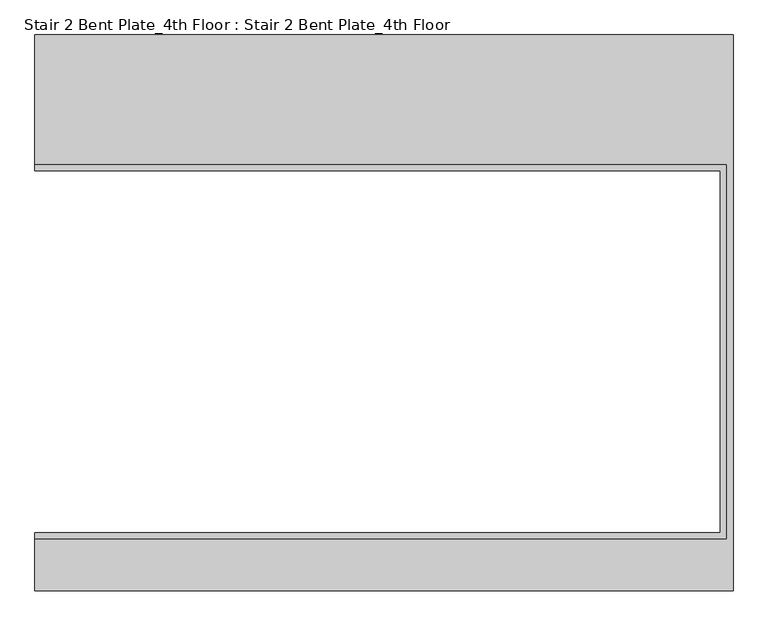
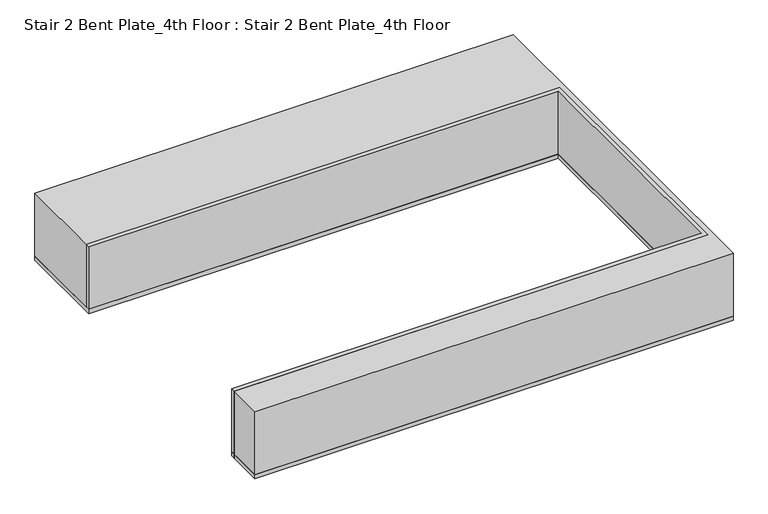
"""IFC4 building model written with IfcOpenShell, lengths in millimetres: proxy geometry, Stair 2 Bent Plate_4th Floor : Stair 2 Bent Plate_4th Floor."""

import ifcopenshell
import ifcopenshell.guid

model = None  # the IFC model being written
_history = None  # IfcOwnerHistory: only IFC2X3 demands one
_inside = {}  # id of a spatial element -> (the spatial element, [elements in it])
_under = {}  # id of a project, library or spatial element -> (it, [spatial elements below it])
_declared = {}  # id of a project -> (the project, [libraries it declares])
_typed = {}  # id of a type object -> (the type object, [elements of that type])
_made_of = {}  # id of a material, layer set ... -> (it, [elements and type objects made of it])


def new_model(schema):
    """Start an empty IFC model of exactly this schema.

    Asked for "IFC4X3", IfcOpenShell would pick the latest addendum, in which some entities
    have other attributes; the version numbers below select the first issue.
    IFC2X3 requires an IfcOwnerHistory on every rooted entity: one is made here for all.
    """
    global model, _history
    if schema == "IFC4X3":
        model = ifcopenshell.file(schema_version=(4, 3, 0, 0))
    else:
        model = ifcopenshell.file(schema=schema)
    _inside.clear()
    _under.clear()
    _declared.clear()
    _typed.clear()
    _made_of.clear()
    _history = None
    if model.schema == "IFC2X3":
        org = make("IfcOrganization", Name="unknown")
        user = make(
            "IfcPersonAndOrganization",
            ThePerson=make("IfcPerson", FamilyName="unknown"),
            TheOrganization=org,
        )
        app = make(
            "IfcApplication",
            ApplicationDeveloper=org,
            Version="unknown",
            ApplicationFullName="unknown",
            ApplicationIdentifier="unknown",
        )
        _history = make(
            "IfcOwnerHistory",
            OwningUser=user,
            OwningApplication=app,
            ChangeAction="ADDED",
            CreationDate=0,
        )
    return model


def make(cls, **values):
    """One entity of the class cls with the attributes given. An attribute that is None is left unset."""
    return model.create_entity(
        cls, **{name: value for name, value in values.items() if value is not None}
    )


def rooted(cls, **values):
    """An entity with a GlobalId (a new one), such as an element, a storey or a relation."""
    return make(cls, GlobalId=ifcopenshell.guid.new(), OwnerHistory=_history, **values)


def si_unit(unit_type, name, prefix=None):
    """IfcSIUnit, for example si_unit("LENGTHUNIT", "METRE", prefix="MILLI")."""
    return make("IfcSIUnit", UnitType=unit_type, Prefix=prefix, Name=name)


def assignment(units):
    """IfcUnitAssignment: the units of a project."""
    return None if units is None else make("IfcUnitAssignment", Units=units)


def point(xyz):
    """IfcCartesianPoint."""
    return None if xyz is None else make("IfcCartesianPoint", Coordinates=xyz)


def direction(xyz):
    """IfcDirection."""
    return None if xyz is None else make("IfcDirection", DirectionRatios=xyz)


def frame(location, z_axis=None, x_axis=None):
    """IfcAxis2Placement3D, a coordinate frame: its origin and axes. An axis left out is left unset."""
    return make(
        "IfcAxis2Placement3D",
        Location=point(location),
        Axis=direction(z_axis),
        RefDirection=direction(x_axis),
    )


def origin():
    """The frame at (0, 0, 0) with its axes left unset."""
    return frame((0.0, 0.0, 0.0))


def origin_with_axes():
    """The frame at (0, 0, 0) with the z axis (0, 0, 1) and the x axis (1, 0, 0) written out."""
    return frame((0.0, 0.0, 0.0), z_axis=(0.0, 0.0, 1.0), x_axis=(1.0, 0.0, 0.0))


def place(relative_to, where):
    """IfcLocalPlacement: puts the frame where relative to a parent placement (None: the world)."""
    return make(
        "IfcLocalPlacement", PlacementRelTo=relative_to, RelativePlacement=where
    )


def context(
    kind, dimensions, precision=None, world=None, true_north=None, identifier=None
):
    """IfcGeometricRepresentationContext, for example the 3D "Model" context."""
    return make(
        "IfcGeometricRepresentationContext",
        ContextIdentifier=identifier,
        ContextType=kind,
        CoordinateSpaceDimension=dimensions,
        Precision=precision,
        WorldCoordinateSystem=world,
        TrueNorth=true_north,
    )


def project(units=None, contexts=None):
    """IfcProject with its units and contexts."""
    return rooted(
        "IfcProject",
        Name="project",
        RepresentationContexts=contexts,
        UnitsInContext=assignment(units),
    )


def spatial(cls, under=None, at=None, **own):
    """A site, building, storey or space (cls), placed at a placement, below another one or the project."""
    s = rooted(cls, ObjectPlacement=at, **own)
    if under is not None:
        _under.setdefault(under.id(), (under, []))[1].append(s)
    return s


def polyline(points):
    """IfcPolyline through the points."""
    return make("IfcPolyline", Points=[point(p) for p in points])


def outline(outer, holes=None, kind="AREA"):
    """IfcArbitraryClosedProfileDef: a profile drawn as a closed curve; with holes, ...WithVoids."""
    if holes is None:
        return make("IfcArbitraryClosedProfileDef", ProfileType=kind, OuterCurve=outer)
    return make(
        "IfcArbitraryProfileDefWithVoids",
        ProfileType=kind,
        OuterCurve=outer,
        InnerCurves=holes,
    )


def extrude(swept, where, along, depth):
    """IfcExtrudedAreaSolid: the profile swept, set in the frame where, extruded along a direction by depth."""
    return make(
        "IfcExtrudedAreaSolid",
        SweptArea=swept,
        Position=where,
        ExtrudedDirection=direction(along),
        Depth=depth,
    )


def shape(context_of_items, identifier, shape_type, items):
    """IfcShapeRepresentation: the items that make up one representation, for example the "Body"."""
    return make(
        "IfcShapeRepresentation",
        ContextOfItems=context_of_items,
        RepresentationIdentifier=identifier,
        RepresentationType=shape_type,
        Items=items,
    )


def source(mapping_origin, context_of_items, identifier, shape_type, items):
    """IfcRepresentationMap: a shape defined once, which mapped items show again and again."""
    return make(
        "IfcRepresentationMap",
        MappingOrigin=mapping_origin,
        MappedRepresentation=shape(context_of_items, identifier, shape_type, items),
    )


def transform(
    local_origin,
    x_axis=None,
    y_axis=None,
    z_axis=None,
    scale=None,
    scale2=None,
    scale3=None,
    uniform=True,
):
    """IfcCartesianTransformationOperator3D, or its non-uniform kind. x_axis, y_axis, z_axis: its Axis1, 2, 3."""
    if uniform:
        return make(
            "IfcCartesianTransformationOperator3D",
            Axis1=direction(x_axis),
            Axis2=direction(y_axis),
            LocalOrigin=point(local_origin),
            Scale=scale,
            Axis3=direction(z_axis),
        )
    return make(
        "IfcCartesianTransformationOperator3DnonUniform",
        Axis1=direction(x_axis),
        Axis2=direction(y_axis),
        LocalOrigin=point(local_origin),
        Scale=scale,
        Axis3=direction(z_axis),
        Scale2=scale2,
        Scale3=scale3,
    )


def mapped(mapping_source, mapping_target):
    """IfcMappedItem: shows the shape of a source again, moved by a transform."""
    return make(
        "IfcMappedItem", MappingSource=mapping_source, MappingTarget=mapping_target
    )


def made_of(thing, what):
    """Note that an element or type object is made of a material, layer set ...; save() writes the relation."""
    if what is not None:
        _made_of.setdefault(what.id(), (what, []))[1].append(thing)
    return thing


def element(
    cls,
    number,
    at=None,
    inside=None,
    cuts=None,
    type_object=None,
    material=None,
    context=None,
    identifier="Body",
    shape_type=None,
    held_by="IfcProductDefinitionShape",
    body=None,
    shapes=None,
    **own,
):
    """One element of the class cls, such as IfcWall. Its Tag is "e" and its number.

    at: its placement. inside: the storey or other place that contains it. cuts: it is an
    opening in that element (IfcRelVoidsElement). A single representation is given by context,
    identifier, shape_type and body (its items); several are given by shapes. held_by: the class
    of the entity that holds the representations. save() writes the other relations.
    """
    e = rooted(cls, Tag="e%d" % number, ObjectPlacement=at, **own)
    if body is not None:
        shapes = [shape(context, identifier, shape_type, body)]
    if shapes is not None:
        e.Representation = make(held_by, Representations=shapes)
    if inside is not None:
        _inside.setdefault(inside.id(), (inside, []))[1].append(e)
    if cuts is not None:
        rooted(
            "IfcRelVoidsElement", RelatingBuildingElement=cuts, RelatedOpeningElement=e
        )
    if type_object is not None:
        _typed.setdefault(type_object.id(), (type_object, []))[1].append(e)
    return made_of(e, material)


def aggregate(whole, parts):
    """IfcRelAggregates: a whole, such as a stair, and the parts it consists of."""
    return rooted("IfcRelAggregates", RelatingObject=whole, RelatedObjects=parts)


def save(model, path):
    """Write the relations noted so far, then the file.

    IfcRelAggregates (storeys below a building ...), IfcRelContainedInSpatialStructure (elements
    in a storey), IfcRelDefinesByType, IfcRelAssociatesMaterial and IfcRelDeclares: one each for
    every whole, place, type object, material and project.
    """
    for whole, parts in _under.values():
        aggregate(whole, parts)
    for where, things in _inside.values():
        rooted(
            "IfcRelContainedInSpatialStructure",
            RelatedElements=things,
            RelatingStructure=where,
        )
    for kind, things in _typed.values():
        rooted("IfcRelDefinesByType", RelatedObjects=things, RelatingType=kind)
    for what, things in _made_of.values():
        rooted("IfcRelAssociatesMaterial", RelatedObjects=things, RelatingMaterial=what)
    for by, libraries in _declared.values():
        rooted("IfcRelDeclares", RelatingContext=by, RelatedDefinitions=libraries)
    model.write(path)


def stair_2_bent_plate_4th_floor_stair_2_bent_plate_4th_floor_69ec89e3(model_context):
    return source(origin(), model_context, "Body", "SweptSolid", [
        extrude(outline(polyline([(-247.65, -815.975), (-247.65, -714.375), (1111.25, -714.375), (1111.25, 22.225), (-247.65, 22.225), (-247.65, 276.225), (1123.95, 276.225), (1123.95, -815.975), (-247.65, -815.975)])), frame((0.0, 0.0, 12.7), z_axis=(0.0, 0.0, 1.0), x_axis=(1.0, 0.0, 0.0)), (0.0, 0.0, 1.0), 190.5),
        extrude(outline(polyline([(1123.95, -815.975), (-247.65, -815.975), (-247.65, -701.675), (1098.55, -701.675), (1098.55, 9.525), (-247.65, 9.525), (-247.65, 276.225), (1123.95, 276.225), (1123.95, -815.975)])), origin_with_axes(), (0.0, 0.0, 1.0), 12.7),
        extrude(outline(polyline([(-247.65, -701.675), (1098.55, -701.675), (1098.55, 9.525), (-247.65, 9.525), (-247.65, 22.225), (1111.25, 22.225), (1111.25, -714.375), (-247.65, -714.375), (-247.65, -701.675)])), origin_with_axes(), (0.0, 0.0, 1.0), 203.2),
    ])


if __name__ == "__main__":
    model = new_model("IFC4")
    model_context = context("Model", 3, world=origin())
    ifc_project = project(units=[si_unit("LENGTHUNIT", "METRE", prefix="MILLI")], contexts=[model_context])
    site = spatial("IfcSite", under=ifc_project)
    building = spatial("IfcBuilding", under=site)
    placement = place(None, origin())
    stair_2_bent_plate_4th_floor_stair_2_bent_plate_4th_floor_shape = stair_2_bent_plate_4th_floor_stair_2_bent_plate_4th_floor_69ec89e3(model_context)
    element("IfcBuildingElementProxy", 1, Name="Stair 2 Bent Plate_4th Floor : Stair 2 Bent Plate_4th Floor", ObjectType="Stair 2 Bent Plate_4th Floor : Stair 2 Bent Plate_4th Floor", at=placement, inside=building, context=model_context, shape_type="MappedRepresentation", body=[
        mapped(stair_2_bent_plate_4th_floor_stair_2_bent_plate_4th_floor_shape, transform((0.0, 0.0, 0.0), x_axis=(1.0, 0.0, 0.0), y_axis=(0.0, 1.0, 0.0), z_axis=(0.0, 0.0, 1.0))),
    ])
    save(model, "model.ifc")

# Revit data of these elements
# Element 1 (IfcBuildingElementProxy, "Stair 2 Bent Plate_4th Floor : Stair 2 Bent Plate_4th Floor")
#   Materials on its faces: "Concrete Infill"
# Materials
#   "Concrete Infill": class "Generic", colour RGB 0 255 0, transparency 0, Cost = 0
